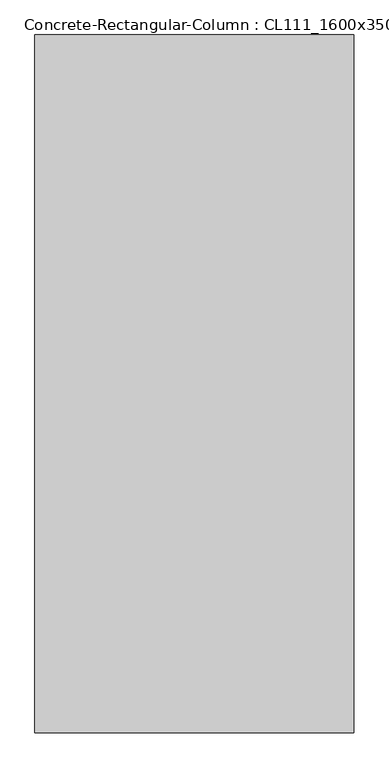
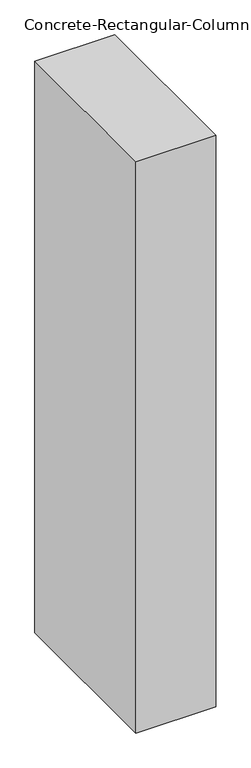
"""IFC4 building model written with IfcOpenShell, lengths in millimetres: column geometry, Concrete-Rectangular-Column : CL111_1600x3500_C1."""

from ifc_helpers import new_model, si_unit, frame, origin, place, context, project, spatial, polyline, outline, extrude, source, transform, mapped, element, save


def concrete_rectangular_column_cl111_1600x3500_c1_e9203d13(model_context):
    return source(origin(), model_context, "Body", "SweptSolid", [
        extrude(outline(polyline([(800.0, 1750.0), (800.0, -1750.0), (-800.0, -1750.0), (-800.0, 1750.0), (800.0, 1750.0)])), frame((0.0, 0.0, -2100.0), z_axis=(0.0, 0.0, 1.0), x_axis=(1.0, 0.0, 0.0)), (0.0, 0.0, 1.0), 12100.0),
    ])


if __name__ == "__main__":
    model = new_model("IFC4")
    model_context = context("Model", 3, world=origin())
    ifc_project = project(units=[si_unit("LENGTHUNIT", "METRE", prefix="MILLI")], contexts=[model_context])
    site = spatial("IfcSite", under=ifc_project)
    building = spatial("IfcBuilding", under=site)
    placement = place(None, origin())
    concrete_rectangular_column_cl111_1600x3500_c1_shape = concrete_rectangular_column_cl111_1600x3500_c1_e9203d13(model_context)
    element("IfcColumn", 1, ObjectType="Concrete-Rectangular-Column : CL111_1600x3500_C1", at=placement, inside=building, context=model_context, shape_type="MappedRepresentation", body=[
        mapped(concrete_rectangular_column_cl111_1600x3500_c1_shape, transform((0.0, 0.0, 0.0), x_axis=(1.0, 0.0, 0.0), y_axis=(0.0, 1.0, 0.0), z_axis=(0.0, 0.0, 1.0))),
    ])
    save(model, "model.ifc")

# Revit data of these elements
# Type "Concrete-Rectangular-Column : CL111_1600x3500_C1"
#   Description = "UG 철골 기둥용 Pedestal"
#   b = 1600 mm
#   h = 3500 mm
#   Width = 1600 mm
#   Length = 3500 mm
#   hec_material3 [instance default] = none
#   hec_material2 [instance default] = A03AE056-00001_Bitumen/Bituminous/Asphalt Coating
#   hec_material1 [instance default] = A03AC035-00001_Form Work (3 times in use)_Flat
#   Structural Material [instance default] = A03AC032-00007_Structural Concrete_Type1_25MPa-30Mpa
# Element 1 (IfcColumn, "Concrete-Rectangular-Column : CL111_1600x3500_C1")
#   hec_material2 = none
#   hec_material1 = none
#   Structural Material = 콘크리트 - 현장타설 콘크리트
#   Materials on its faces: "콘크리트 - 현장타설 콘크리트"
# Materials
#   "A03AE056-00001_Bitumen/Bituminous/Asphalt Coating": class "Generic", colour RGB 17 17 17, transparency 0, Description = "Damp-proofing", W00) Work Master Code = "A03AE056-00001", W01) Work Master_Lv1 = "Concrete Work", W02) Work Master_Lv2 = "Concrete Protective Coating (U/G)", W03) Work Master_Spec.1 = "Bitumen/Bituminous/Asphalt Coating", Cost = 0
#   "A03AC035-00001_Form Work (3 times in use)_Flat": class "Wood", colour RGB 149 120 74, transparency 0, Description = "Plywood", W00) Work Master Code = "A03AC035-00001", W01) Work Master_Lv1 = "Concrete Work", W02) Work Master_Lv2 = "Substructure Work", W03) Work Master_Spec.1 = "Form Work (3 times in use)", W04) Work Master_Spec.2 = "Flat Form", W05) Work Master_Spec.3 = "Dressed Lumber, Plywood or Steel Form(Wood Planks are not Allowed) incl. Chamfer", Cost = 0
#   "A03AC032-00007_Structural Concrete_Type1_25MPa-30Mpa": class "Concrete", colour RGB 176 176 176, transparency 0, Keynote = "09910.A1", Description = "Reinf. Conc.", W00) Work Master Code = "A03AC032-00007", W01) Work Master_Lv1 = "Concrete Work", W02) Work Master_Lv2 = "Substructure Work", W03) Work Master_Spec.1 = "Structural Concrete", W04) Work Master_Spec.2 = "Cement Type-1", W05) Work Master_Spec.3 = "25MPa < F'c (Cylinder Strength) ≤ 30MPa", Cost = 0
#   "콘크리트 - 현장타설 콘크리트": class "콘크리트", colour RGB 192 192 192, transparency 0
